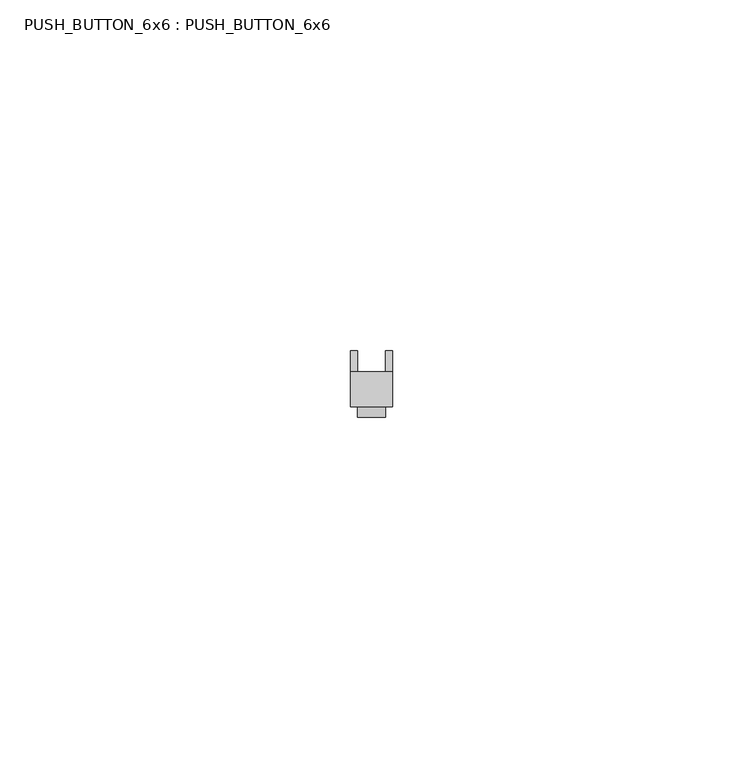
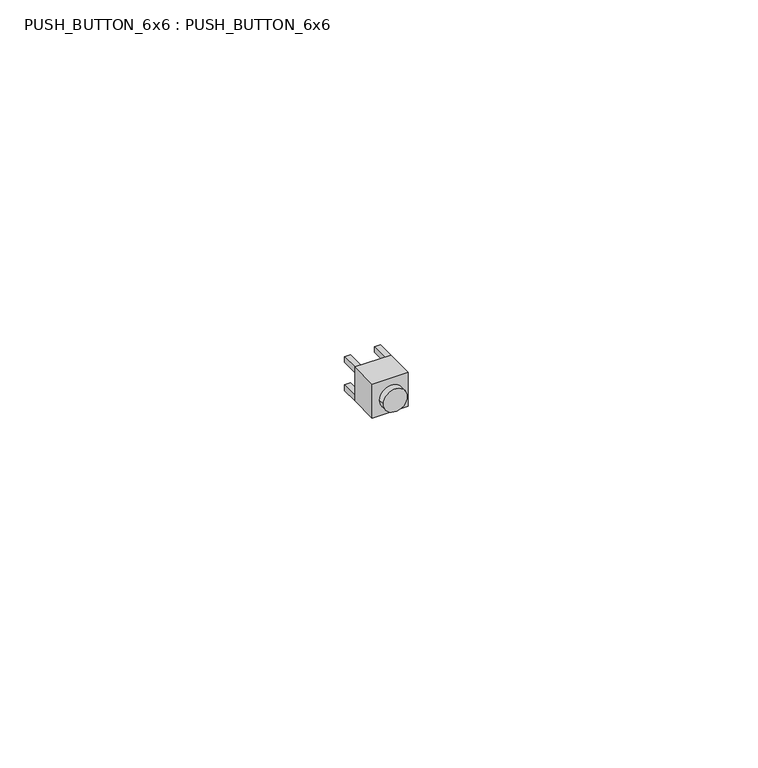
"""IFC4 building model written with IfcOpenShell, lengths in millimetres: furniture geometry, PUSH_BUTTON_6x6 : PUSH_BUTTON_6x6."""

from ifc_helpers import new_model, si_unit, point, frame, frame_2d, origin, origin_with_axes, place, context, project, spatial, polyline, circle_curve, trimmed, segment, composite_curve, outline, extrude, source, transform, mapped, element, save


def push_button_6x6_push_button_6x6_b47c84f7(model_context):
    return source(origin(), model_context, "Body", "SweptSolid", [
        extrude(outline(polyline([(-3.0, 0.0), (-3.0, 5.0), (3.0, 5.0), (3.0, 0.0), (-3.0, 0.0)])), origin_with_axes(), (0.0, 0.0, 1.0), 6.0),
        extrude(outline(composite_curve([segment(trimmed(circle_curve(frame_2d((3.0, 0.0)), 2.0), [point((3.0, -2.0))], [point((3.0, 2.0))], False, "CARTESIAN"), True, "CONTINUOUS"), segment(trimmed(circle_curve(frame_2d((3.0, 0.0)), 2.0), [point((3.0, 2.0))], [point((3.0, -2.0))], False, "CARTESIAN"), True, "CONTINUOUS")], self_intersect=False)), frame((0.0, -1.5, 0.0), z_axis=(0.0, 1.0, 0.0), x_axis=(0.0, 0.0, 1.0)), (0.0, 0.0, 1.0), 1.5),
        extrude(outline(polyline([(3.0, 5.0), (2.0, 5.0), (2.0, 8.0), (3.0, 8.0), (3.0, 5.0)])), frame((0.0, 0.0, 5.0), z_axis=(0.0, 0.0, 1.0), x_axis=(1.0, 0.0, 0.0)), (0.0, 0.0, 1.0), 1.0),
        extrude(outline(polyline([(-2.0, 5.0), (-3.0, 5.0), (-3.0, 8.0), (-2.0, 8.0), (-2.0, 5.0)])), frame((0.0, 0.0, 5.0), z_axis=(0.0, 0.0, 1.0), x_axis=(1.0, 0.0, 0.0)), (0.0, 0.0, 1.0), 1.0),
        extrude(outline(polyline([(3.0, 5.0), (2.0, 5.0), (2.0, 8.0), (3.0, 8.0), (3.0, 5.0)])), origin_with_axes(), (0.0, 0.0, 1.0), 1.0),
        extrude(outline(polyline([(-2.0, 5.0), (-3.0, 5.0), (-3.0, 8.0), (-2.0, 8.0), (-2.0, 5.0)])), origin_with_axes(), (0.0, 0.0, 1.0), 1.0),
    ])


if __name__ == "__main__":
    model = new_model("IFC4")
    model_context = context("Model", 3, world=origin())
    ifc_project = project(units=[si_unit("LENGTHUNIT", "METRE", prefix="MILLI")], contexts=[model_context])
    site = spatial("IfcSite", under=ifc_project)
    building = spatial("IfcBuilding", under=site)
    placement = place(None, origin())
    push_button_6x6_push_button_6x6_shape = push_button_6x6_push_button_6x6_b47c84f7(model_context)
    element("IfcFurniture", 1, ObjectType="PUSH_BUTTON_6x6 : PUSH_BUTTON_6x6", at=placement, inside=building, context=model_context, shape_type="MappedRepresentation", body=[
        mapped(push_button_6x6_push_button_6x6_shape, transform((0.0, 0.0, 0.0), x_axis=(1.0, 0.0, 0.0), y_axis=(0.0, 1.0, 0.0), z_axis=(0.0, 0.0, 1.0))),
    ])
    save(model, "model.ifc")

# Revit data of these elements
# Type "PUSH_BUTTON_6x6 : PUSH_BUTTON_6x6"
#   Default Elevation = 0
# Element 1 (IfcFurniture, "PUSH_BUTTON_6x6 : PUSH_BUTTON_6x6")
#   Materials on its faces: ".BOTAO"
# Materials
#   ".BOTAO": class "Vidro", colour RGB 0 255 255, transparency 0.75, Cost = 0
